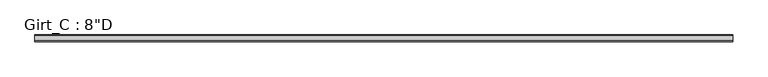
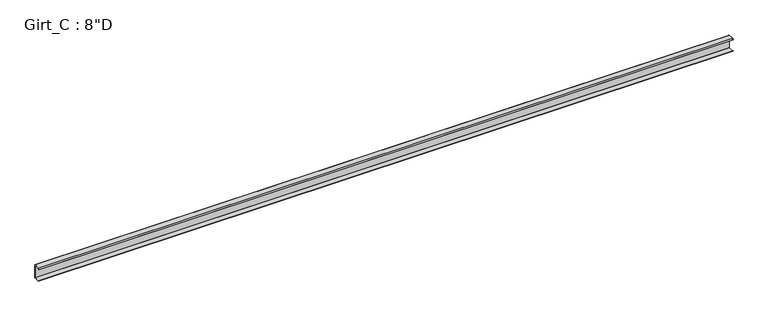
"""IFC4 building model written with IfcOpenShell, lengths in millimetres: beam geometry."""

from ifc_helpers import new_model, si_unit, point, frame, frame_2d, origin, place, context, project, spatial, polyline, circle_curve, trimmed, segment, composite_curve, outline, extrude, source, transform, mapped, element, save


def beam_db347ce0(model_context):
    return source(origin(), model_context, "Body", "SweptSolid", [
        extrude(outline(composite_curve([segment(polyline([(-87.5109375, 101.6), (-3.3734375, 101.6)]), True, "CONTINUOUS"), segment(trimmed(circle_curve(frame_2d((-3.3734375, 96.8375)), 4.7625), [point((-3.3734375, 101.6))], [point((1.3890625, 96.8375))], False, "CARTESIAN"), True, "CONTINUOUS"), segment(polyline([(1.3890625, 96.8375), (1.3890625, -96.8375)]), True, "CONTINUOUS"), segment(trimmed(circle_curve(frame_2d((-3.3734375, -96.8375)), 4.7625), [point((1.3890625, -96.8375))], [point((-3.3734375, -101.6))], False, "CARTESIAN"), True, "CONTINUOUS"), segment(polyline([(-3.3734375, -101.6), (-87.5109375, -101.6), (-99.7792647, -86.979177), (-97.6510975, -85.1934327), (-86.2154765, -98.821875), (-3.2694106, -98.821875)]), True, "CONTINUOUS"), segment(trimmed(circle_curve(frame_2d((-3.3748024, -96.8389339)), 1.9857399), [point((-3.2694106, -98.821875))], [point((-1.3890625, -96.8389339))], True, "CARTESIAN"), True, "CONTINUOUS"), segment(polyline([(-1.3890625, -96.8389339), (-1.3890625, 96.8381931)]), True, "CONTINUOUS"), segment(trimmed(circle_curve(frame_2d((-3.3741066, 96.8381931)), 1.9850441), [point((-1.3890625, 96.8381931))], [point((-3.3005807, 98.821875))], True, "CARTESIAN"), True, "CONTINUOUS"), segment(polyline([(-3.3005807, 98.821875), (-86.2154765, 98.821875), (-97.6278742, 85.221109), (-99.7560415, 87.0068534), (-87.5109375, 101.6)]), True, "CONTINUOUS")], self_intersect=False)), frame((-5126.2407, 0.0, 0.0), z_axis=(1.0, 0.0, 0.0), x_axis=(0.0, 1.0, 0.0)), (0.0, 0.0, 1.0), 10266.553),
    ])


if __name__ == "__main__":
    model = new_model("IFC4")
    model_context = context("Model", 3, world=origin())
    ifc_project = project(units=[si_unit("LENGTHUNIT", "METRE", prefix="MILLI")], contexts=[model_context])
    site = spatial("IfcSite", under=ifc_project)
    building = spatial("IfcBuilding", under=site)
    placement = place(None, origin())
    beam_shape = beam_db347ce0(model_context)
    element("IfcBeam", 1, ObjectType="Girt_C : 8\"D", at=placement, inside=building, context=model_context, shape_type="MappedRepresentation", body=[
        mapped(beam_shape, transform((0.0, 0.0, 0.0), x_axis=(1.0, 0.0, 0.0), y_axis=(0.0, 1.0, 0.0), z_axis=(0.0, 0.0, 1.0))),
    ])
    save(model, "model.ifc")

# Revit data of these elements
# Type "Girt_C : 8\"D"
#   half leg = 0' - 1 3/4"
#   Web_Thickness = 0' - 0 7/64"
#   Length [instance default] = 10' - 0"
#   Leg_1 = 0' - 3 1/2"
#   Height = 0' - 8"
#   Structural Material [instance default] = none
# Element 1 (IfcBeam, "Girt_C : 8\"D")
#   Materials on its faces: "CEE' SECTION (8.0x3.5C - SEE STRUCT. DWGS)"
# Materials
#   "CEE' SECTION (8.0x3.5C - SEE STRUCT. DWGS)": class "Metal", colour RGB 137 146 153, transparency 0, Description = "Steel, mill finish", Cost = 0
